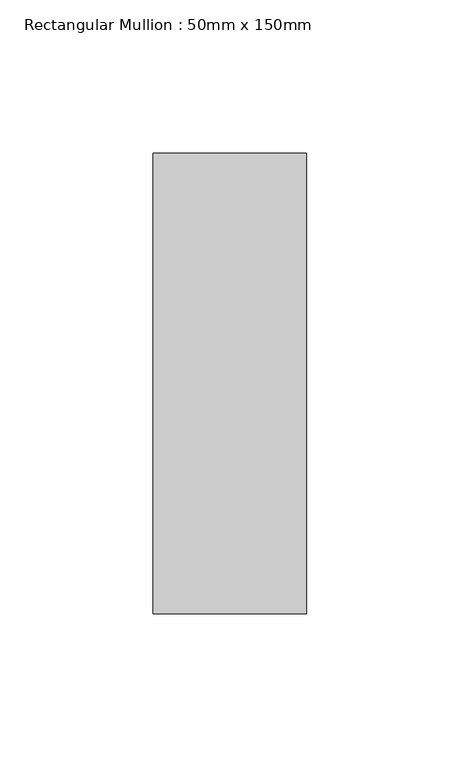
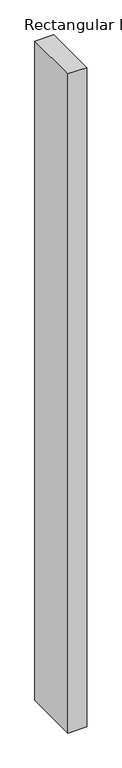
"""IFC4 building model written with IfcOpenShell, lengths in millimetres: member geometry, Rectangular Mullion : 50mm x 150mm."""

from ifc_helpers import new_model, si_unit, frame, origin, place, context, project, spatial, polyline, outline, extrude, source, transform, mapped, element, save


def rectangular_mullion_50mm_x_150mm_42770ee2(model_context):
    return source(origin(), model_context, "Body", "SweptSolid", [
        extrude(outline(polyline([(0.0, 75.0), (0.0, -75.0), (-50.0, -75.0), (-50.0, 75.0), (0.0, 75.0)])), frame((0.0, 0.0, -1830.0000003), z_axis=(0.0, 0.0, 1.0), x_axis=(1.0, 0.0, 0.0)), (0.0, 0.0, 1.0), 1830.0000003),
    ])


if __name__ == "__main__":
    model = new_model("IFC4")
    model_context = context("Model", 3, world=origin())
    ifc_project = project(units=[si_unit("LENGTHUNIT", "METRE", prefix="MILLI")], contexts=[model_context])
    site = spatial("IfcSite", under=ifc_project)
    building = spatial("IfcBuilding", under=site)
    placement = place(None, origin())
    rectangular_mullion_50mm_x_150mm_shape = rectangular_mullion_50mm_x_150mm_42770ee2(model_context)
    element("IfcMember", 1, ObjectType="Rectangular Mullion : 50mm x 150mm", at=placement, inside=building, context=model_context, shape_type="MappedRepresentation", body=[
        mapped(rectangular_mullion_50mm_x_150mm_shape, transform((0.0, 0.0, 0.0), x_axis=(1.0, 0.0, 0.0), y_axis=(0.0, 1.0, 0.0), z_axis=(0.0, 0.0, 1.0))),
    ])
    save(model, "model.ifc")

# Revit data of these elements
# Type "Rectangular Mullion : 50mm x 150mm"
#   built-in parameter 1007304 = 0.492126 (stored number, unit not read)
#   built-in parameter 1007301 = 0.082021 (stored number, unit not read)
#   built-in parameter 1007300 = 0.082021 (stored number, unit not read)
# Element 1 (IfcMember, "Rectangular Mullion : 50mm x 150mm")
#   Materials on its faces: "Aluminum"
# Materials
#   "Aluminum": class "Metal", colour RGB 244 244 244, transparency 0, Description = "Aluminum 6061", Cost = 0
